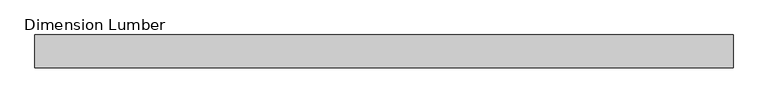
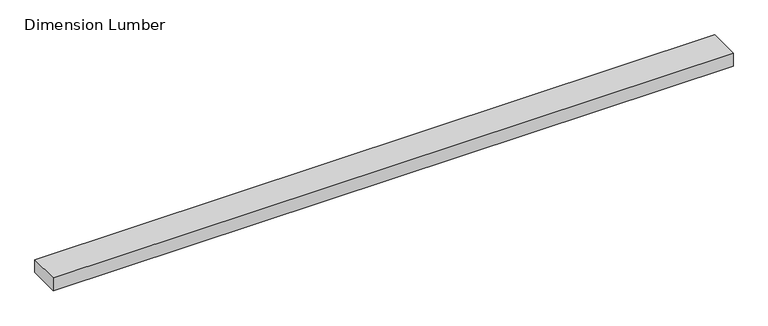
"""IFC4 building model written with IfcOpenShell, lengths in millimetres: beam geometry, Dimension Lumber : Top Supporting Lumbers."""

from ifc_helpers import new_model, si_unit, frame, origin, place, context, project, spatial, polyline, outline, extrude, source, transform, mapped, element, save


def dimension_lumber_72c26da1(model_context):
    return source(origin(), model_context, "Body", "SweptSolid", [
        extrude(outline(polyline([(927.1, 44.45), (927.1, -44.45), (-971.55, -44.45), (-971.55, 44.45), (927.1, 44.45)])), frame((0.0, 0.0, -19.05), z_axis=(0.0, 0.0, 1.0), x_axis=(1.0, 0.0, 0.0)), (0.0, 0.0, 1.0), 38.1),
    ])


if __name__ == "__main__":
    model = new_model("IFC4")
    model_context = context("Model", 3, world=origin())
    ifc_project = project(units=[si_unit("LENGTHUNIT", "METRE", prefix="MILLI")], contexts=[model_context])
    site = spatial("IfcSite", under=ifc_project)
    building = spatial("IfcBuilding", under=site)
    placement = place(None, origin())
    dimension_lumber_shape = dimension_lumber_72c26da1(model_context)
    element("IfcBeam", 1, ObjectType="Dimension Lumber : Top Supporting Lumbers", at=placement, inside=building, context=model_context, shape_type="MappedRepresentation", body=[
        mapped(dimension_lumber_shape, transform((0.0, 0.0, 0.0), x_axis=(1.0, 0.0, 0.0), y_axis=(0.0, 1.0, 0.0), z_axis=(0.0, 0.0, 1.0))),
    ])
    save(model, "model.ifc")

# Revit data of these elements
# Type "Dimension Lumber : Top Supporting Lumbers"
#   Assembly Code = "B10"
#   A = 0.0364583 SF
#   Length [instance default] = 5' - 0"
#   b = 0' - 3 1/2"
#   d = 0' - 1 1/2"
#   Structural Material [instance default] = Softwood, Lumber
# Element 1 (IfcBeam, "Dimension Lumber : Top Supporting Lumbers")
#   Structural Material = Douglas Fir #2
#   Materials on its faces: "Douglas Fir #2"
# Materials
#   "Softwood, Lumber": class "Wood", colour RGB 223 192 134, transparency 0, Description = "Pinus Echinata", Cost = 0
#   "Douglas Fir #2": class "Wood", colour RGB 223 192 134, transparency 0, Description = "Pinus Echinata", Cost = 0
